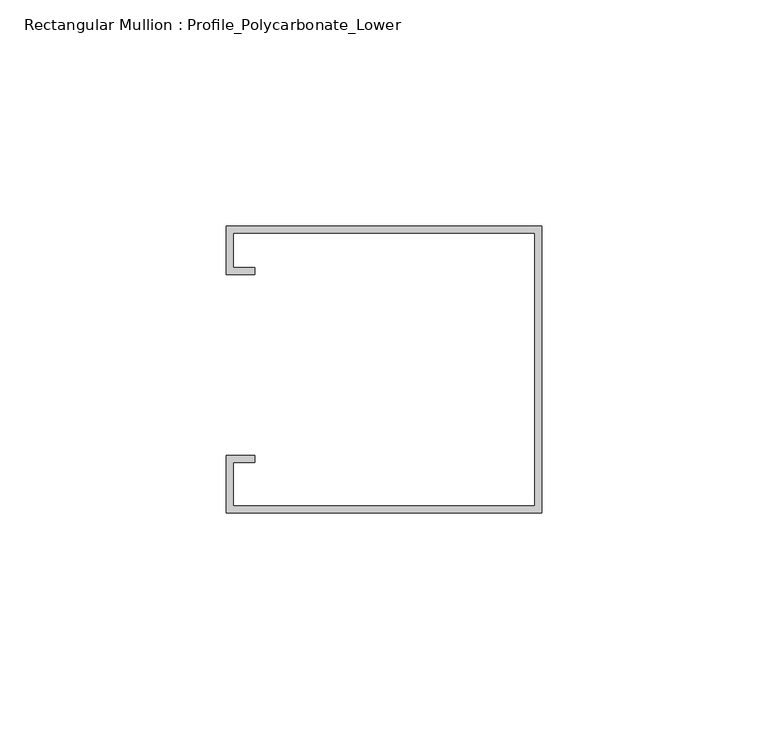
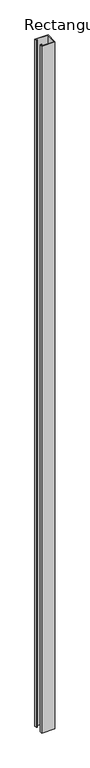
"""IFC4 building model written with IfcOpenShell, lengths in millimetres: member geometry, Rectangular Mullion : Profile_Polycarbonate_Lower."""

from ifc_helpers import new_model, si_unit, frame, origin, place, context, project, spatial, polyline, outline, extrude, source, transform, mapped, element, save


def rectangular_mullion_profile_polycarbonate_lower_ada87149(model_context):
    return source(origin(), model_context, "Body", "SweptSolid", [
        extrude(outline(polyline([(0.0, -32.7), (-69.85, -32.7), (-69.85, -20.0), (-63.5, -20.0), (-63.5, -21.5875), (-68.2625, -21.5875), (-68.2625, -31.1125), (-1.5875, -31.1125), (-1.5875, 29.2125), (-68.2625, 29.2125), (-68.2625, 21.5875), (-63.5, 21.5875), (-63.5, 20.0), (-69.85, 20.0), (-69.85, 30.8), (0.0, 30.8), (0.0, -32.7)])), frame((0.0, 0.0, -3871.275), z_axis=(0.0, 0.0, 1.0), x_axis=(1.0, 0.0, 0.0)), (0.0, 0.0, 1.0), 3871.275),
    ])


if __name__ == "__main__":
    model = new_model("IFC4")
    model_context = context("Model", 3, world=origin())
    ifc_project = project(units=[si_unit("LENGTHUNIT", "METRE", prefix="MILLI")], contexts=[model_context])
    site = spatial("IfcSite", under=ifc_project)
    building = spatial("IfcBuilding", under=site)
    placement = place(None, origin())
    rectangular_mullion_profile_polycarbonate_lower_shape = rectangular_mullion_profile_polycarbonate_lower_ada87149(model_context)
    element("IfcMember", 1, ObjectType="Rectangular Mullion : Profile_Polycarbonate_Lower", at=placement, inside=building, context=model_context, shape_type="MappedRepresentation", body=[
        mapped(rectangular_mullion_profile_polycarbonate_lower_shape, transform((0.0, 0.0, 0.0), x_axis=(1.0, 0.0, 0.0), y_axis=(0.0, 1.0, 0.0), z_axis=(0.0, 0.0, 1.0))),
    ])
    save(model, "model.ifc")

# Revit data of these elements
# Type "Rectangular Mullion : Profile_Polycarbonate_Lower"
#   built-in parameter 1007322 = 0.208333 (stored number, unit not read)
#   built-in parameter 1007321 = 0 (stored number, unit not read)
#   built-in parameter 1007320 = 0.00520833 (stored number, unit not read)
# Element 1 (IfcMember, "Rectangular Mullion : Profile_Polycarbonate_Lower")
#   Materials on its faces: "Aluminum"
# Materials
#   "Aluminum": class "Metal", colour RGB 244 244 244, transparency 0, Description = "Aluminum 6061", Cost = 0
